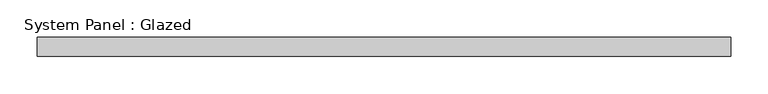
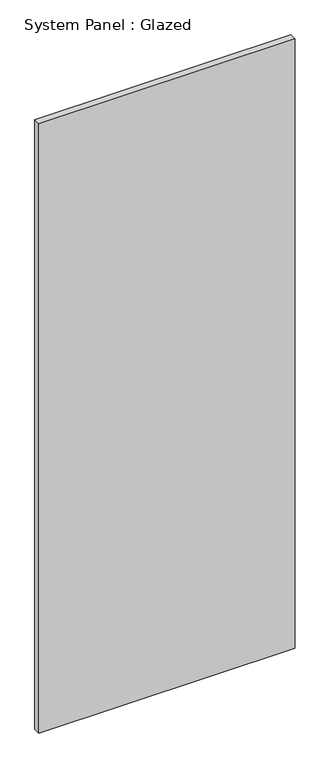
"""IFC4 building model written with IfcOpenShell, lengths in millimetres: plate geometry, System Panel : Glazed."""

import ifcopenshell
import ifcopenshell.guid

model = None  # the IFC model being written
_history = None  # IfcOwnerHistory: only IFC2X3 demands one
_inside = {}  # id of a spatial element -> (the spatial element, [elements in it])
_under = {}  # id of a project, library or spatial element -> (it, [spatial elements below it])
_declared = {}  # id of a project -> (the project, [libraries it declares])
_typed = {}  # id of a type object -> (the type object, [elements of that type])
_made_of = {}  # id of a material, layer set ... -> (it, [elements and type objects made of it])


def new_model(schema):
    """Start an empty IFC model of exactly this schema.

    Asked for "IFC4X3", IfcOpenShell would pick the latest addendum, in which some entities
    have other attributes; the version numbers below select the first issue.
    IFC2X3 requires an IfcOwnerHistory on every rooted entity: one is made here for all.
    """
    global model, _history
    if schema == "IFC4X3":
        model = ifcopenshell.file(schema_version=(4, 3, 0, 0))
    else:
        model = ifcopenshell.file(schema=schema)
    _inside.clear()
    _under.clear()
    _declared.clear()
    _typed.clear()
    _made_of.clear()
    _history = None
    if model.schema == "IFC2X3":
        org = make("IfcOrganization", Name="unknown")
        user = make(
            "IfcPersonAndOrganization",
            ThePerson=make("IfcPerson", FamilyName="unknown"),
            TheOrganization=org,
        )
        app = make(
            "IfcApplication",
            ApplicationDeveloper=org,
            Version="unknown",
            ApplicationFullName="unknown",
            ApplicationIdentifier="unknown",
        )
        _history = make(
            "IfcOwnerHistory",
            OwningUser=user,
            OwningApplication=app,
            ChangeAction="ADDED",
            CreationDate=0,
        )
    return model


def make(cls, **values):
    """One entity of the class cls with the attributes given. An attribute that is None is left unset."""
    return model.create_entity(
        cls, **{name: value for name, value in values.items() if value is not None}
    )


def rooted(cls, **values):
    """An entity with a GlobalId (a new one), such as an element, a storey or a relation."""
    return make(cls, GlobalId=ifcopenshell.guid.new(), OwnerHistory=_history, **values)


def si_unit(unit_type, name, prefix=None):
    """IfcSIUnit, for example si_unit("LENGTHUNIT", "METRE", prefix="MILLI")."""
    return make("IfcSIUnit", UnitType=unit_type, Prefix=prefix, Name=name)


def assignment(units):
    """IfcUnitAssignment: the units of a project."""
    return None if units is None else make("IfcUnitAssignment", Units=units)


def point(xyz):
    """IfcCartesianPoint."""
    return None if xyz is None else make("IfcCartesianPoint", Coordinates=xyz)


def direction(xyz):
    """IfcDirection."""
    return None if xyz is None else make("IfcDirection", DirectionRatios=xyz)


def frame(location, z_axis=None, x_axis=None):
    """IfcAxis2Placement3D, a coordinate frame: its origin and axes. An axis left out is left unset."""
    return make(
        "IfcAxis2Placement3D",
        Location=point(location),
        Axis=direction(z_axis),
        RefDirection=direction(x_axis),
    )


def origin():
    """The frame at (0, 0, 0) with its axes left unset."""
    return frame((0.0, 0.0, 0.0))


def origin_with_axes():
    """The frame at (0, 0, 0) with the z axis (0, 0, 1) and the x axis (1, 0, 0) written out."""
    return frame((0.0, 0.0, 0.0), z_axis=(0.0, 0.0, 1.0), x_axis=(1.0, 0.0, 0.0))


def place(relative_to, where):
    """IfcLocalPlacement: puts the frame where relative to a parent placement (None: the world)."""
    return make(
        "IfcLocalPlacement", PlacementRelTo=relative_to, RelativePlacement=where
    )


def context(
    kind, dimensions, precision=None, world=None, true_north=None, identifier=None
):
    """IfcGeometricRepresentationContext, for example the 3D "Model" context."""
    return make(
        "IfcGeometricRepresentationContext",
        ContextIdentifier=identifier,
        ContextType=kind,
        CoordinateSpaceDimension=dimensions,
        Precision=precision,
        WorldCoordinateSystem=world,
        TrueNorth=true_north,
    )


def project(units=None, contexts=None):
    """IfcProject with its units and contexts."""
    return rooted(
        "IfcProject",
        Name="project",
        RepresentationContexts=contexts,
        UnitsInContext=assignment(units),
    )


def spatial(cls, under=None, at=None, **own):
    """A site, building, storey or space (cls), placed at a placement, below another one or the project."""
    s = rooted(cls, ObjectPlacement=at, **own)
    if under is not None:
        _under.setdefault(under.id(), (under, []))[1].append(s)
    return s


def polyline(points):
    """IfcPolyline through the points."""
    return make("IfcPolyline", Points=[point(p) for p in points])


def outline(outer, holes=None, kind="AREA"):
    """IfcArbitraryClosedProfileDef: a profile drawn as a closed curve; with holes, ...WithVoids."""
    if holes is None:
        return make("IfcArbitraryClosedProfileDef", ProfileType=kind, OuterCurve=outer)
    return make(
        "IfcArbitraryProfileDefWithVoids",
        ProfileType=kind,
        OuterCurve=outer,
        InnerCurves=holes,
    )


def extrude(swept, where, along, depth):
    """IfcExtrudedAreaSolid: the profile swept, set in the frame where, extruded along a direction by depth."""
    return make(
        "IfcExtrudedAreaSolid",
        SweptArea=swept,
        Position=where,
        ExtrudedDirection=direction(along),
        Depth=depth,
    )


def shape(context_of_items, identifier, shape_type, items):
    """IfcShapeRepresentation: the items that make up one representation, for example the "Body"."""
    return make(
        "IfcShapeRepresentation",
        ContextOfItems=context_of_items,
        RepresentationIdentifier=identifier,
        RepresentationType=shape_type,
        Items=items,
    )


def source(mapping_origin, context_of_items, identifier, shape_type, items):
    """IfcRepresentationMap: a shape defined once, which mapped items show again and again."""
    return make(
        "IfcRepresentationMap",
        MappingOrigin=mapping_origin,
        MappedRepresentation=shape(context_of_items, identifier, shape_type, items),
    )


def transform(
    local_origin,
    x_axis=None,
    y_axis=None,
    z_axis=None,
    scale=None,
    scale2=None,
    scale3=None,
    uniform=True,
):
    """IfcCartesianTransformationOperator3D, or its non-uniform kind. x_axis, y_axis, z_axis: its Axis1, 2, 3."""
    if uniform:
        return make(
            "IfcCartesianTransformationOperator3D",
            Axis1=direction(x_axis),
            Axis2=direction(y_axis),
            LocalOrigin=point(local_origin),
            Scale=scale,
            Axis3=direction(z_axis),
        )
    return make(
        "IfcCartesianTransformationOperator3DnonUniform",
        Axis1=direction(x_axis),
        Axis2=direction(y_axis),
        LocalOrigin=point(local_origin),
        Scale=scale,
        Axis3=direction(z_axis),
        Scale2=scale2,
        Scale3=scale3,
    )


def mapped(mapping_source, mapping_target):
    """IfcMappedItem: shows the shape of a source again, moved by a transform."""
    return make(
        "IfcMappedItem", MappingSource=mapping_source, MappingTarget=mapping_target
    )


def made_of(thing, what):
    """Note that an element or type object is made of a material, layer set ...; save() writes the relation."""
    if what is not None:
        _made_of.setdefault(what.id(), (what, []))[1].append(thing)
    return thing


def element(
    cls,
    number,
    at=None,
    inside=None,
    cuts=None,
    type_object=None,
    material=None,
    context=None,
    identifier="Body",
    shape_type=None,
    held_by="IfcProductDefinitionShape",
    body=None,
    shapes=None,
    **own,
):
    """One element of the class cls, such as IfcWall. Its Tag is "e" and its number.

    at: its placement. inside: the storey or other place that contains it. cuts: it is an
    opening in that element (IfcRelVoidsElement). A single representation is given by context,
    identifier, shape_type and body (its items); several are given by shapes. held_by: the class
    of the entity that holds the representations. save() writes the other relations.
    """
    e = rooted(cls, Tag="e%d" % number, ObjectPlacement=at, **own)
    if body is not None:
        shapes = [shape(context, identifier, shape_type, body)]
    if shapes is not None:
        e.Representation = make(held_by, Representations=shapes)
    if inside is not None:
        _inside.setdefault(inside.id(), (inside, []))[1].append(e)
    if cuts is not None:
        rooted(
            "IfcRelVoidsElement", RelatingBuildingElement=cuts, RelatedOpeningElement=e
        )
    if type_object is not None:
        _typed.setdefault(type_object.id(), (type_object, []))[1].append(e)
    return made_of(e, material)


def aggregate(whole, parts):
    """IfcRelAggregates: a whole, such as a stair, and the parts it consists of."""
    return rooted("IfcRelAggregates", RelatingObject=whole, RelatedObjects=parts)


def save(model, path):
    """Write the relations noted so far, then the file.

    IfcRelAggregates (storeys below a building ...), IfcRelContainedInSpatialStructure (elements
    in a storey), IfcRelDefinesByType, IfcRelAssociatesMaterial and IfcRelDeclares: one each for
    every whole, place, type object, material and project.
    """
    for whole, parts in _under.values():
        aggregate(whole, parts)
    for where, things in _inside.values():
        rooted(
            "IfcRelContainedInSpatialStructure",
            RelatedElements=things,
            RelatingStructure=where,
        )
    for kind, things in _typed.values():
        rooted("IfcRelDefinesByType", RelatedObjects=things, RelatingType=kind)
    for what, things in _made_of.values():
        rooted("IfcRelAssociatesMaterial", RelatedObjects=things, RelatingMaterial=what)
    for by, libraries in _declared.values():
        rooted("IfcRelDeclares", RelatingContext=by, RelatedDefinitions=libraries)
    model.write(path)


def system_panel_glazed_70154507(model_context):
    return source(origin(), model_context, "Body", "SweptSolid", [
        extrude(outline(polyline([(462.5, 24.5), (-462.5, 24.5), (-462.5, 49.5), (462.5, 49.5), (462.5, 24.5)])), origin_with_axes(), (0.0, 0.0, 1.0), 2325.0),
    ])


if __name__ == "__main__":
    model = new_model("IFC4")
    model_context = context("Model", 3, world=origin())
    ifc_project = project(units=[si_unit("LENGTHUNIT", "METRE", prefix="MILLI")], contexts=[model_context])
    site = spatial("IfcSite", under=ifc_project)
    building = spatial("IfcBuilding", under=site)
    placement = place(None, origin())
    system_panel_glazed_shape = system_panel_glazed_70154507(model_context)
    element("IfcPlate", 1, ObjectType="System Panel : Glazed", at=placement, inside=building, context=model_context, shape_type="MappedRepresentation", body=[
        mapped(system_panel_glazed_shape, transform((0.0, 0.0, 0.0), x_axis=(1.0, 0.0, 0.0), y_axis=(0.0, 1.0, 0.0), z_axis=(0.0, 0.0, 1.0))),
    ])
    save(model, "model.ifc")

# Revit data of these elements
# Type "System Panel : Glazed"
#   Construction Type Id = "GSP4R"
#   Analytic Construction = "1/8 in Pilkington single glazing"
#   Visual Light Transmittance = 0.9
#   Solar Heat Gain Coefficient = 0.86
#   Heat Transfer Coefficient (U) = 6.7069 W/(m²·K)
#   Define Thermal Properties by = 1
# Element 1 (IfcPlate, "System Panel : Glazed")
#   Materials on its faces: "Glass"
# Materials
#   "Glass": class "Glass", colour RGB 0 128 192, transparency 0.9, Description = "Soda Lime Glass", Cost = 0
